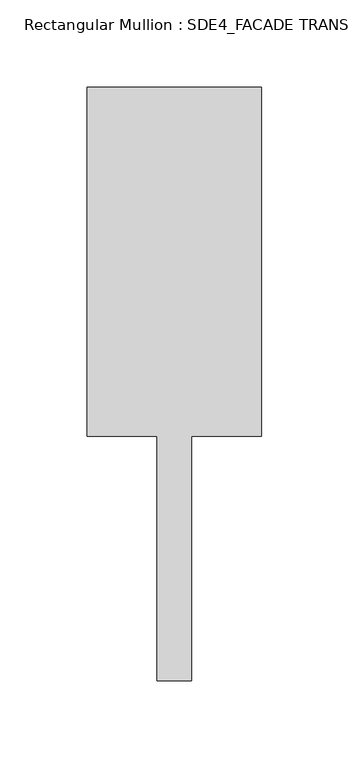
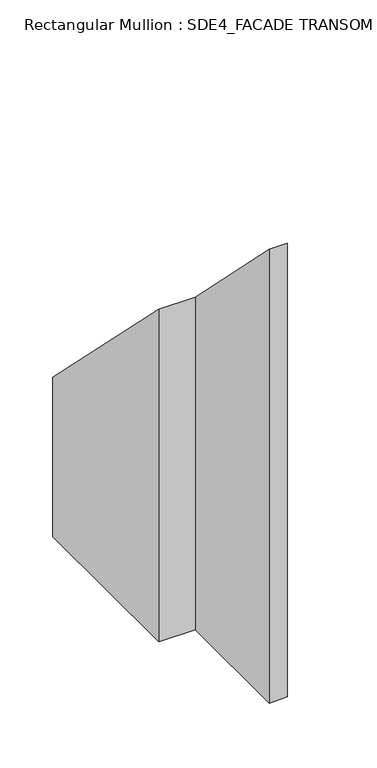
"""IFC4 building model written with IfcOpenShell, lengths in millimetres: member geometry, Rectangular Mullion : SDE4_FACADE TRANSOM TYPE 1."""

from ifc_helpers import new_model, si_unit, origin, place, context, project, spatial, faceted_brep, source, transform, mapped, element, save


def rectangular_mullion_sde4_facade_transom_type_1_5f5cd1cd(model_context):
    return source(origin(), model_context, "Body", "Brep", [
        faceted_brep([(50.0, 132.5, -316.4624711), (50.0, -67.5, -316.4624711), (10.0, -67.5, -316.4624711), (10.0, -207.5, -316.4624711), (-10.0, -207.5, -316.4624711), (-10.0, -67.5, -316.4624711), (-50.0, -67.5, -316.4624711), (-50.0, 132.5, -316.4624711), (-50.0, 132.5, -132.5), (50.0, 132.5, -132.5), (-50.0, -67.5, 67.5), (-10.0, -67.5, 67.5), (-10.0, -207.5, 207.5), (10.0, -207.5, 207.5), (10.0, -67.5, 67.5), (50.0, -67.5, 67.5)], [[[0, 1, 2, 3, 4, 5, 6, 7]], [[8, 9, 0, 7]], [[10, 8, 7, 6]], [[11, 10, 6, 5]], [[12, 11, 5, 4]], [[13, 12, 4, 3]], [[14, 13, 3, 2]], [[15, 14, 2, 1]], [[9, 15, 1, 0]], [[9, 8, 10, 11, 12, 13, 14, 15]]]),
    ])


if __name__ == "__main__":
    model = new_model("IFC4")
    model_context = context("Model", 3, world=origin())
    ifc_project = project(units=[si_unit("LENGTHUNIT", "METRE", prefix="MILLI")], contexts=[model_context])
    site = spatial("IfcSite", under=ifc_project)
    building = spatial("IfcBuilding", under=site)
    placement = place(None, origin())
    rectangular_mullion_sde4_facade_transom_type_1_shape = rectangular_mullion_sde4_facade_transom_type_1_5f5cd1cd(model_context)
    element("IfcMember", 1, ObjectType="Rectangular Mullion : SDE4_FACADE TRANSOM TYPE 1", at=placement, inside=building, context=model_context, shape_type="MappedRepresentation", body=[
        mapped(rectangular_mullion_sde4_facade_transom_type_1_shape, transform((0.0, 0.0, 0.0), x_axis=(1.0, 0.0, 0.0), y_axis=(0.0, 1.0, 0.0), z_axis=(0.0, 0.0, 1.0))),
    ])
    save(model, "model.ifc")

# Revit data of these elements
# Type "Rectangular Mullion : SDE4_FACADE TRANSOM TYPE 1"
#   built-in parameter 1007322 = 1.11549 (stored number, unit not read)
#   built-in parameter 1007321 = 0.164042 (stored number, unit not read)
#   built-in parameter 1007320 = 0.164042 (stored number, unit not read)
